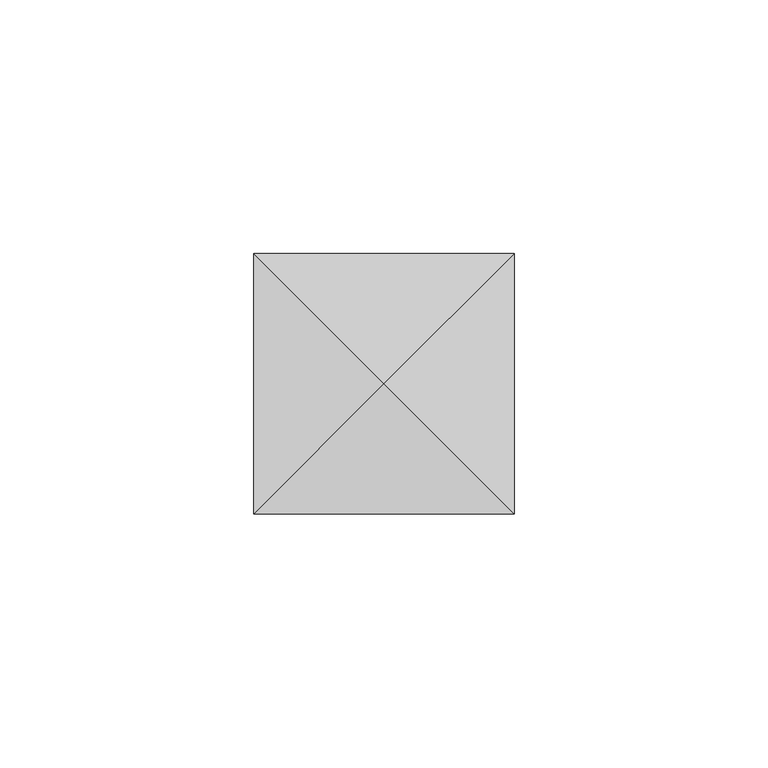
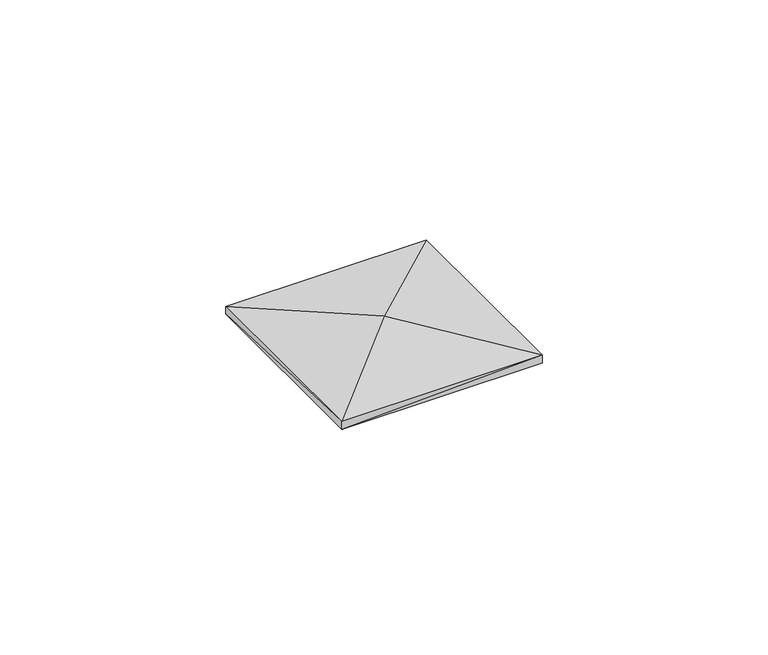
"""IFC4 building model written with IfcOpenShell, lengths in millimetres: geographic element geometry, Enscape AssetDefinition - Flower 024 Dandelion Flower (leaves) : Enscape AssetDefinition - Flower 024 Dandelion Flower (leaves)."""

from ifc_helpers import new_model, si_unit, origin, place, context, project, spatial, faceted_brep, source, transform, mapped, element, save


def geographic_element_fa8c9055(model_context):
    return source(origin(), model_context, "Body", "Brep", [
        faceted_brep([(25.7263519, 25.7263519, 0.0), (-25.7263519, -25.7263519, 0.0), (-25.7263519, 25.7263519, 0.0), (25.7263519, -25.7263519, 0.0), (-25.7263519, 25.7263519, 2.0581081), (0.0, 0.0, 6.0304548), (25.7263519, 25.7263519, 2.0581081), (25.7263519, -25.7263519, 2.0581081), (-25.7263519, -25.7263519, 2.0581081)], [[[0, 1, 2]], [[1, 0, 3]], [[4, 5, 6]], [[7, 1, 3]], [[1, 7, 8]], [[6, 3, 0]], [[3, 6, 7]], [[4, 0, 2]], [[0, 4, 6]], [[8, 2, 1]], [[2, 8, 4]], [[5, 7, 6]], [[5, 4, 8]], [[7, 5, 8]]]),
    ])


if __name__ == "__main__":
    model = new_model("IFC4")
    model_context = context("Model", 3, world=origin())
    ifc_project = project(units=[si_unit("LENGTHUNIT", "METRE", prefix="MILLI")], contexts=[model_context])
    site = spatial("IfcSite", under=ifc_project)
    building = spatial("IfcBuilding", under=site)
    placement = place(None, origin())
    geographic_element_shape = geographic_element_fa8c9055(model_context)
    element("IfcGeographicElement", 1, ObjectType="Enscape AssetDefinition - Flower 024 Dandelion Flower (leaves) : Enscape AssetDefinition - Flower 024 Dandelion Flower (leaves)", at=placement, inside=building, context=model_context, shape_type="MappedRepresentation", body=[
        mapped(geographic_element_shape, transform((0.0, 0.0, 0.0), x_axis=(1.0, 0.0, 0.0), y_axis=(0.0, 1.0, 0.0), z_axis=(0.0, 0.0, 1.0))),
    ])
    save(model, "model.ifc")

# Revit data of these elements
# Type "Enscape AssetDefinition - Flower 024 Dandelion Flower (leaves) : Enscape AssetDefinition - Flower 024 Dandelion Flower (leaves)"
#   EnscapeAssetSource = "REMOTE"
#   EnscapeAssetId = "a4e79c13-3098-4cc5-8423-8b5aff9cc4b1"
#   Height = 0.00603 m
#   EnscapeNativeAssetHeight = 0.00603 m
#   Default Elevation = 0
